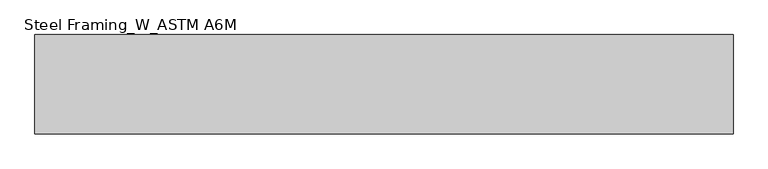
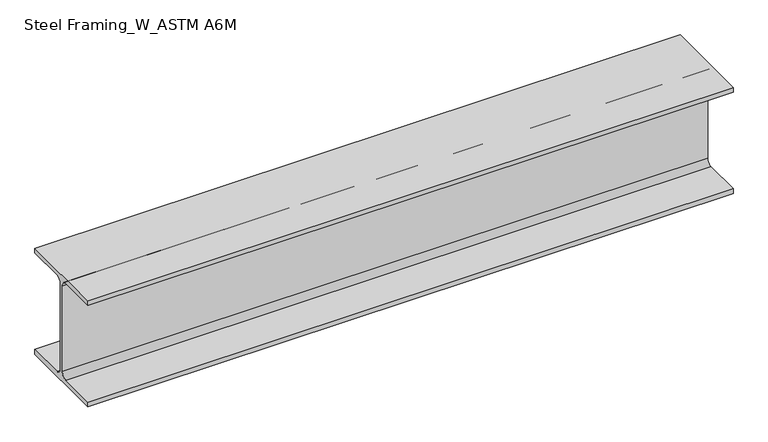
"""IFC4 building model written with IfcOpenShell, lengths in millimetres: beam geometry, Steel Framing_W_ASTM A6M : H_SB_AR_S02_W250x49.1_G5."""

from ifc_helpers import new_model, si_unit, point, frame, frame_2d, origin, place, context, project, spatial, polyline, circle_curve, trimmed, segment, composite_curve, outline, extrude, source, transform, mapped, element, save


def steel_framing_w_astm_a6m_e7a7b24c(model_context):
    return source(origin(), model_context, "Body", "SweptSolid", [
        extrude(outline(composite_curve([segment(polyline([(101.0, -112.5), (101.0, -123.5), (-101.0, -123.5), (-101.0, -112.5), (-16.385, -112.5)]), True, "CONTINUOUS"), segment(trimmed(circle_curve(frame_2d((-16.385, -99.8)), 12.7), [point((-16.385, -112.5))], [point((-3.685, -99.8))], True, "CARTESIAN"), True, "CONTINUOUS"), segment(polyline([(-3.685, -99.8), (-3.685, 99.8)]), True, "CONTINUOUS"), segment(trimmed(circle_curve(frame_2d((-16.385, 99.8)), 12.7), [point((-3.685, 99.8))], [point((-16.385, 112.5))], True, "CARTESIAN"), True, "CONTINUOUS"), segment(polyline([(-16.385, 112.5), (-101.0, 112.5), (-101.0, 123.5), (101.0, 123.5), (101.0, 112.5), (16.385, 112.5)]), True, "CONTINUOUS"), segment(trimmed(circle_curve(frame_2d((16.385, 99.8)), 12.7), [point((16.385, 112.5))], [point((3.685, 99.8))], True, "CARTESIAN"), True, "CONTINUOUS"), segment(polyline([(3.685, 99.8), (3.685, -99.8)]), True, "CONTINUOUS"), segment(trimmed(circle_curve(frame_2d((16.385, -99.8)), 12.7), [point((3.685, -99.8))], [point((16.385, -112.5))], True, "CARTESIAN"), True, "CONTINUOUS"), segment(polyline([(16.385, -112.5), (101.0, -112.5)]), True, "CONTINUOUS")], self_intersect=False)), frame((-553.8, 0.0, 0.0), z_axis=(1.0, 0.0, 0.0), x_axis=(0.0, 1.0, 0.0)), (0.0, 0.0, 1.0), 1420.8),
    ])


if __name__ == "__main__":
    model = new_model("IFC4")
    model_context = context("Model", 3, world=origin())
    ifc_project = project(units=[si_unit("LENGTHUNIT", "METRE", prefix="MILLI")], contexts=[model_context])
    site = spatial("IfcSite", under=ifc_project)
    building = spatial("IfcBuilding", under=site)
    placement = place(None, origin())
    steel_framing_w_astm_a6m_shape = steel_framing_w_astm_a6m_e7a7b24c(model_context)
    element("IfcBeam", 1, ObjectType="Steel Framing_W_ASTM A6M : H_SB_AR_S02_W250x49.1_G5", at=placement, inside=building, context=model_context, shape_type="MappedRepresentation", body=[
        mapped(steel_framing_w_astm_a6m_shape, transform((0.0, 0.0, 0.0), x_axis=(1.0, 0.0, 0.0), y_axis=(0.0, 1.0, 0.0), z_axis=(0.0, 0.0, 1.0))),
    ])
    save(model, "model.ifc")

# Revit data of these elements
# Type "Steel Framing_W_ASTM A6M : H_SB_AR_S02_W250x49.1_G5"
#   Type Mark = "G5"
#   Section Name Key = "W10x33"
#   Width = 20.2 cm
#   Web Thickness = 0.737 cm
#   Web Fillet = 1.27 cm
#   Warping Constant = 212000.0 cm⁶
#   Torsional Moment of Inertia = 24.30 cm⁴
#   Section Area = 62.6 cm²
#   Plastic Modulus weak axis = 229.0 cm³
#   Plastic Modulus strong axis = 636.0 cm³
#   Perimeter = 1.27 m²/m
#   Nominal Weight = 49.10 kgf/m
#   Moment of Inertia weak axis = 1520.00 cm⁴
#   Moment of Inertia strong axis = 7120.00 cm⁴
#   Height = 24.7 cm
#   Flange Thickness = 1.1 cm
#   Elastic Modulus weak axis = 151.0 cm³
#   Elastic Modulus strong axis = 574.0 cm³
#   Centroid Vertical = 12.35 cm
#   Centroid Horizontal = 10.1 cm
#   Length [instance default] = 1500 mm
#   Structural Material [instance default] = Steel, 45-345
#   Bolt Spacing = 0
#   Assembly Code = ""
# Element 1 (IfcBeam, "Steel Framing_W_ASTM A6M : H_SB_AR_S02_W250x49.1_G5")
#   Materials on its faces: "Steel, 45-345"
# Materials
#   "Steel, 45-345": class "Metal", colour RGB 189 187 185, transparency 0, Description = "Steel 345 MPa", Cost = 0
